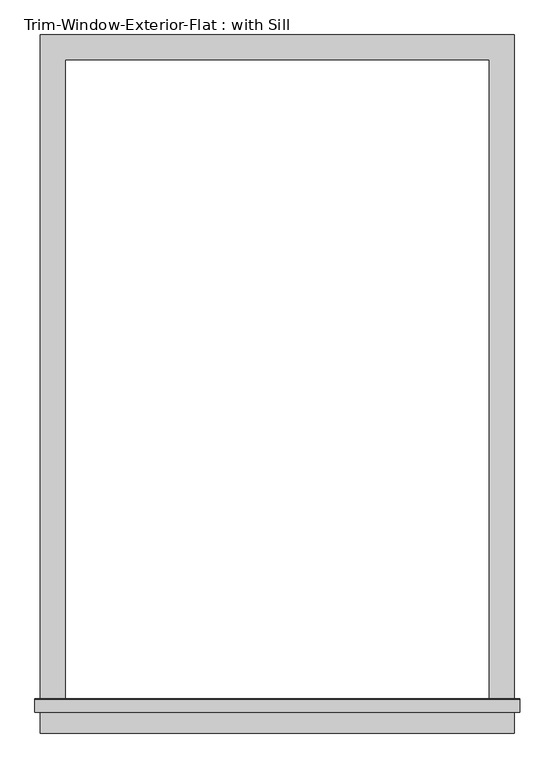
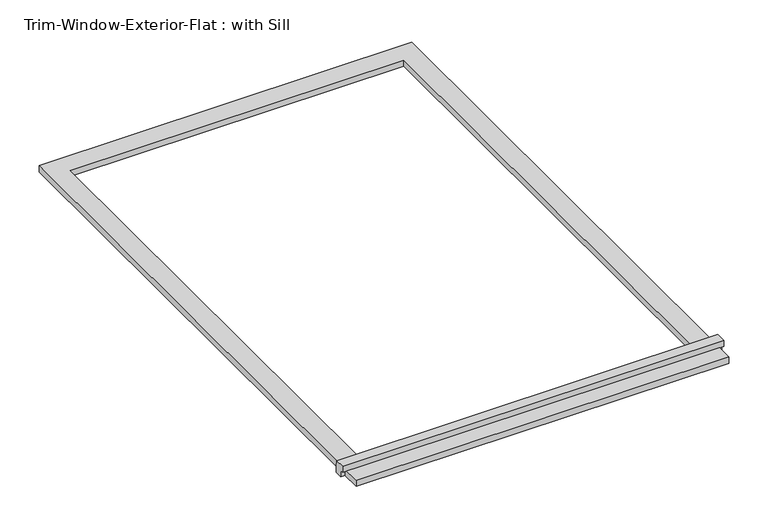
"""IFC4 building model written with IfcOpenShell, lengths in millimetres: proxy geometry, Trim-Window-Exterior-Flat : with Sill."""

from ifc_helpers import new_model, si_unit, frame, origin, origin_with_axes, place, context, project, spatial, polyline, outline, extrude, source, transform, mapped, element, save


def trim_window_exterior_flat_with_sill_6766514a(model_context):
    return source(origin(), model_context, "Body", "SweptSolid", [
        extrude(outline(polyline([(546.1, -1495.3823709), (546.1, -1552.5323709), (-546.1, -1552.5323709), (-546.1, -1495.3823709), (546.1, -1495.3823709)])), origin_with_axes(), (0.0, 0.0, 1.0), 19.05),
        extrude(outline(polyline([(-1504.95, 38.1), (-1475.6580645, 38.1), (-1473.2, 19.05), (-1473.2, 0.0), (-1495.3823709, 0.0), (-1495.3823709, 19.05), (-1504.95, 19.05), (-1504.95, 38.1)])), frame((-558.8, 0.0, 0.0), z_axis=(1.0, 0.0, 0.0), x_axis=(0.0, 1.0, 0.0)), (0.0, 0.0, 1.0), 1117.6),
        extrude(outline(polyline([(-546.1, 57.15), (546.1, 57.15), (546.1, -1473.2), (488.95, -1473.2), (488.95, 0.0), (-488.95, 0.0), (-488.95, -1473.2), (-546.1, -1473.2), (-546.1, 57.15)])), origin_with_axes(), (0.0, 0.0, 1.0), 19.05),
    ])


if __name__ == "__main__":
    model = new_model("IFC4")
    model_context = context("Model", 3, world=origin())
    ifc_project = project(units=[si_unit("LENGTHUNIT", "METRE", prefix="MILLI")], contexts=[model_context])
    site = spatial("IfcSite", under=ifc_project)
    building = spatial("IfcBuilding", under=site)
    placement = place(None, origin())
    trim_window_exterior_flat_with_sill_shape = trim_window_exterior_flat_with_sill_6766514a(model_context)
    element("IfcBuildingElementProxy", 1, Name="Trim-Window-Exterior-Flat : with Sill", ObjectType="Trim-Window-Exterior-Flat : with Sill", at=placement, inside=building, context=model_context, shape_type="MappedRepresentation", body=[
        mapped(trim_window_exterior_flat_with_sill_shape, transform((0.0, 0.0, 0.0), x_axis=(1.0, 0.0, 0.0), y_axis=(0.0, 1.0, 0.0), z_axis=(0.0, 0.0, 1.0))),
    ])
    save(model, "model.ifc")

# Revit data of these elements
# Type "Trim-Window-Exterior-Flat : with Sill"
#   Trim Width = 0' - 2 1/4"
#   Trim Thickness_Picture Frame = 0' - 1 1/4"
#   Trim Thickness_with Sill = 0' - 0 3/4"
#   Sill Thickness = 0' - 1 1/4"
#   Opening Width [instance default] = 2' - 0"
#   Opening Height [instance default] = 3' - 0"
#   Default Elevation = 4' - 0"
#   Sill = yes
#   Picture Frame = no
#   Trim Material [instance default] = none
# Element 1 (IfcBuildingElementProxy, "Trim-Window-Exterior-Flat : with Sill")
#   Opening Width = 3' - 2 1/2"
#   Opening Height = 4' - 10"
#   Trim Material = 1X WOOD COMPOSITE TRIM
#   Materials on its faces: "1X WOOD COMPOSITE TRIM"
# Materials
#   "1X WOOD COMPOSITE TRIM": class "Generic", colour RGB 88 61 61, transparency 0, Cost = 0
